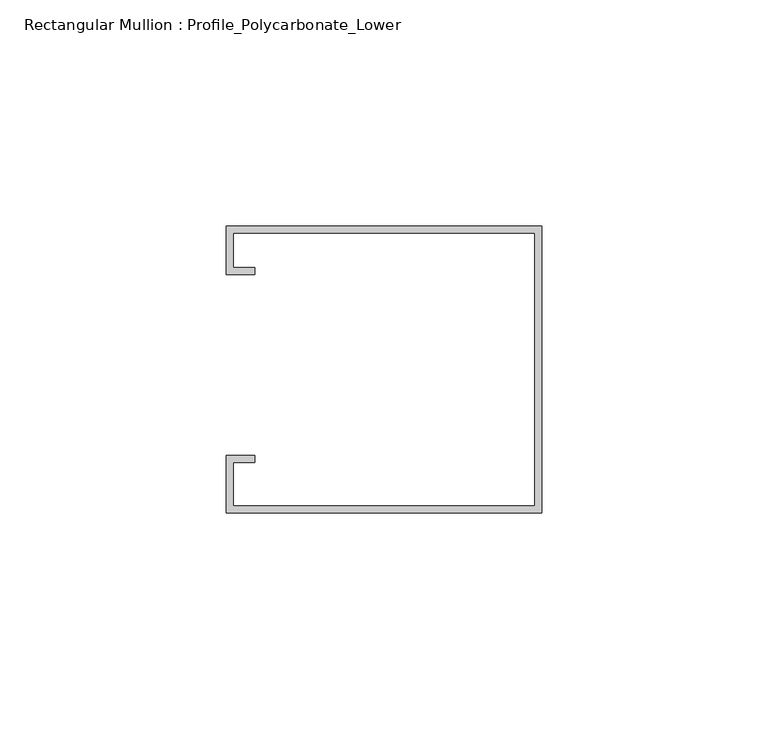
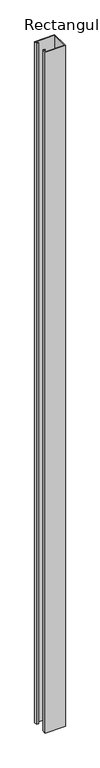
"""IFC4 building model written with IfcOpenShell, lengths in millimetres: member geometry, Rectangular Mullion : Profile_Polycarbonate_Lower."""

from ifc_helpers import new_model, si_unit, frame, origin, place, context, project, spatial, polyline, outline, extrude, source, transform, mapped, element, save


def rectangular_mullion_profile_polycarbonate_lower_0f329726(model_context):
    return source(origin(), model_context, "Body", "SweptSolid", [
        extrude(outline(polyline([(0.0, -32.7), (-69.85, -32.7), (-69.85, -20.0), (-63.5, -20.0), (-63.5, -21.5875), (-68.2625, -21.5875), (-68.2625, -31.1125), (-1.5875, -31.1125), (-1.5875, 29.2125), (-68.2625, 29.2125), (-68.2625, 21.5875), (-63.5, 21.5875), (-63.5, 20.0), (-69.85, 20.0), (-69.85, 30.8), (0.0, 30.8), (0.0, -32.7)])), frame((0.0, 0.0, -2505.075), z_axis=(0.0, 0.0, 1.0), x_axis=(1.0, 0.0, 0.0)), (0.0, 0.0, 1.0), 2505.075),
    ])


if __name__ == "__main__":
    model = new_model("IFC4")
    model_context = context("Model", 3, world=origin())
    ifc_project = project(units=[si_unit("LENGTHUNIT", "METRE", prefix="MILLI")], contexts=[model_context])
    site = spatial("IfcSite", under=ifc_project)
    building = spatial("IfcBuilding", under=site)
    placement = place(None, origin())
    rectangular_mullion_profile_polycarbonate_lower_shape = rectangular_mullion_profile_polycarbonate_lower_0f329726(model_context)
    element("IfcMember", 1, ObjectType="Rectangular Mullion : Profile_Polycarbonate_Lower", at=placement, inside=building, context=model_context, shape_type="MappedRepresentation", body=[
        mapped(rectangular_mullion_profile_polycarbonate_lower_shape, transform((0.0, 0.0, 0.0), x_axis=(1.0, 0.0, 0.0), y_axis=(0.0, 1.0, 0.0), z_axis=(0.0, 0.0, 1.0))),
    ])
    save(model, "model.ifc")

# Revit data of these elements
# Type "Rectangular Mullion : Profile_Polycarbonate_Lower"
#   built-in parameter 1007322 = 0.208333 (stored number, unit not read)
#   built-in parameter 1007321 = 0 (stored number, unit not read)
#   built-in parameter 1007320 = 0.00520833 (stored number, unit not read)
# Element 1 (IfcMember, "Rectangular Mullion : Profile_Polycarbonate_Lower")
#   Materials on its faces: "ALUMINUM PROFILE AT POLYCARBONATE PANEL"
# Materials
#   "ALUMINUM PROFILE AT POLYCARBONATE PANEL": class "Metal", colour RGB 244 244 244, transparency 0, Description = "Aluminum 6061", Cost = 0
